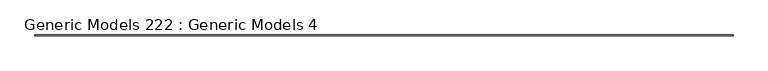
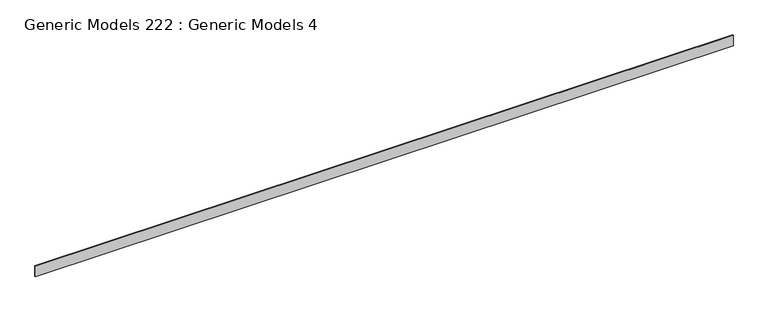
"""IFC4 building model written with IfcOpenShell, lengths in millimetres: proxy geometry, Generic Models 222 : Generic Models 4."""

from ifc_helpers import new_model, si_unit, frame, origin, place, context, project, spatial, polyline, outline, extrude, source, transform, mapped, element, save


def generic_models_222_generic_models_4_beb8de19(model_context):
    return source(origin(), model_context, "Body", "SweptSolid", [
        extrude(outline(polyline([(-2152.1733045, -29321.7235482), (-2152.1733045, -29340.7735482), (-20795.7733045, -29340.7735482), (-20795.7733045, -29321.7235482), (-2152.1733045, -29321.7235482)])), frame((0.0, 0.0, 126841.091198), z_axis=(0.0, 0.0, 1.0), x_axis=(1.0, 0.0, 0.0)), (0.0, 0.0, 1.0), 290.0279303),
    ])


if __name__ == "__main__":
    model = new_model("IFC4")
    model_context = context("Model", 3, world=origin())
    ifc_project = project(units=[si_unit("LENGTHUNIT", "METRE", prefix="MILLI")], contexts=[model_context])
    site = spatial("IfcSite", under=ifc_project)
    building = spatial("IfcBuilding", under=site)
    placement = place(None, origin())
    generic_models_222_generic_models_4_shape = generic_models_222_generic_models_4_beb8de19(model_context)
    element("IfcBuildingElementProxy", 1, Name="Generic Models 222 : Generic Models 4", ObjectType="Generic Models 222 : Generic Models 4", at=placement, inside=building, context=model_context, shape_type="MappedRepresentation", body=[
        mapped(generic_models_222_generic_models_4_shape, transform((0.0, 0.0, 0.0), x_axis=(1.0, 0.0, 0.0), y_axis=(0.0, 1.0, 0.0), z_axis=(0.0, 0.0, 1.0))),
    ])
    save(model, "model.ifc")

# Revit data of these elements
# Element 1 (IfcBuildingElementProxy, "Generic Models 222 : Generic Models 4")
#   Materials on its faces: "_CDX PLYWOOD - SEE STRUCT DWGs"
# Materials
#   "_CDX PLYWOOD - SEE STRUCT DWGs": class "Generic", colour RGB 98 75 74, transparency 0, Cost = 0
